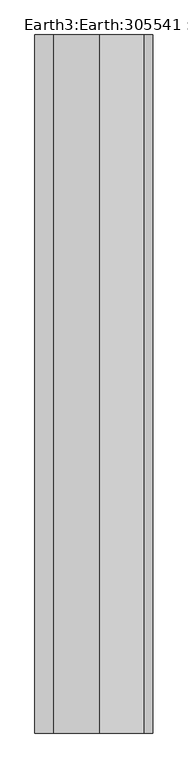
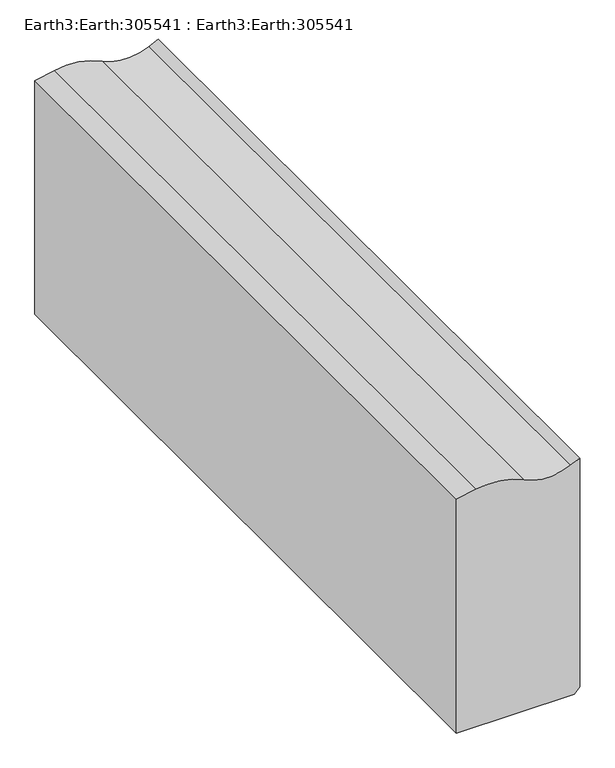
"""IFC4 building model written with IfcOpenShell, lengths in millimetres: proxy geometry, Earth3:Earth:305541 : Earth3:Earth:305541."""

from ifc_helpers import new_model, si_unit, point, frame, frame_2d, origin, place, context, project, spatial, polyline, circle_curve, trimmed, segment, composite_curve, outline, extrude, source, transform, mapped, element, save


def earth3_earth_305541_earth3_earth_305541_580bc910(model_context):
    return source(origin(), model_context, "Body", "SweptSolid", [
        extrude(outline(composite_curve([segment(polyline([(33311.3426943, -5268.4580306), (32634.014262, -5268.4580306), (32634.014262, -4946.142691), (32649.5954298, -4930.5615232), (33312.2775477, -4930.5615232), (33300.0908366, -4956.8836877)]), True, "CONTINUOUS"), segment(trimmed(circle_curve(frame_2d((33431.3167137, -5017.6390203)), 144.607888), [point((33300.0908366, -4956.8836877))], [point((33302.6181918, -5083.5793852))], True, "CARTESIAN"), True, "CONTINUOUS"), segment(trimmed(circle_curve(frame_2d((33120.1913863, -5177.0481363)), 204.9779178), [point((33302.6181918, -5083.5793852))], [point((33321.4784396, -5215.7711136))], False, "CARTESIAN"), True, "CONTINUOUS"), segment(polyline([(33321.4784396, -5215.7711136), (33311.3426943, -5268.4580306)]), True, "CONTINUOUS")], self_intersect=False)), frame((0.0, 7460.4857132, 0.0), z_axis=(0.0, 1.0, 0.0), x_axis=(0.0, 0.0, 1.0)), (0.0, 0.0, 1.0), 2000.0),
    ])


if __name__ == "__main__":
    model = new_model("IFC4")
    model_context = context("Model", 3, world=origin())
    ifc_project = project(units=[si_unit("LENGTHUNIT", "METRE", prefix="MILLI")], contexts=[model_context])
    site = spatial("IfcSite", under=ifc_project)
    building = spatial("IfcBuilding", under=site)
    placement = place(None, origin())
    earth3_earth_305541_earth3_earth_305541_shape = earth3_earth_305541_earth3_earth_305541_580bc910(model_context)
    element("IfcBuildingElementProxy", 1, Name="Earth3:Earth:305541 : Earth3:Earth:305541", ObjectType="Earth3:Earth:305541 : Earth3:Earth:305541", at=placement, inside=building, context=model_context, shape_type="MappedRepresentation", body=[
        mapped(earth3_earth_305541_earth3_earth_305541_shape, transform((0.0, 0.0, 0.0), x_axis=(1.0, 0.0, 0.0), y_axis=(0.0, 1.0, 0.0), z_axis=(0.0, 0.0, 1.0))),
    ])
    save(model, "model.ifc")

# Revit data of these elements
# Type "Earth3:Earth:305541 : Earth3:Earth:305541"
#   NameOverride = "Earth3:Earth:305541"
#   ObjectTypeOverride = "Earth3:Earth"
#   Reference = "Earth"
#   Category = "Generic Models"
#   Tag = "305541"
# Element 1 (IfcBuildingElementProxy, "Earth3:Earth:305541 : Earth3:Earth:305541")
#   Materials on its faces: "GROUND SOIL"
# Materials
#   "GROUND SOIL": class "Unassigned", colour RGB 170 124 75, transparency 0, Cost = 0
